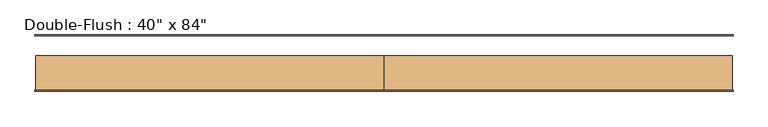
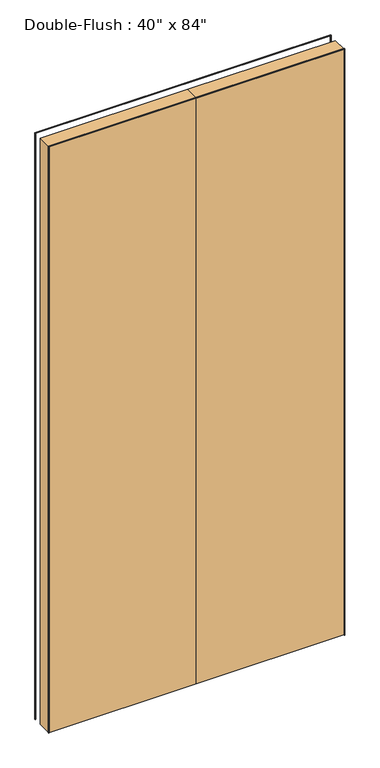
"""IFC4 building model written with IfcOpenShell, lengths in millimetres: door geometry."""

import ifcopenshell
import ifcopenshell.guid

model = None  # the IFC model being written
_history = None  # IfcOwnerHistory: only IFC2X3 demands one
_inside = {}  # id of a spatial element -> (the spatial element, [elements in it])
_under = {}  # id of a project, library or spatial element -> (it, [spatial elements below it])
_declared = {}  # id of a project -> (the project, [libraries it declares])
_typed = {}  # id of a type object -> (the type object, [elements of that type])
_made_of = {}  # id of a material, layer set ... -> (it, [elements and type objects made of it])


def new_model(schema):
    """Start an empty IFC model of exactly this schema.

    Asked for "IFC4X3", IfcOpenShell would pick the latest addendum, in which some entities
    have other attributes; the version numbers below select the first issue.
    IFC2X3 requires an IfcOwnerHistory on every rooted entity: one is made here for all.
    """
    global model, _history
    if schema == "IFC4X3":
        model = ifcopenshell.file(schema_version=(4, 3, 0, 0))
    else:
        model = ifcopenshell.file(schema=schema)
    _inside.clear()
    _under.clear()
    _declared.clear()
    _typed.clear()
    _made_of.clear()
    _history = None
    if model.schema == "IFC2X3":
        org = make("IfcOrganization", Name="unknown")
        user = make(
            "IfcPersonAndOrganization",
            ThePerson=make("IfcPerson", FamilyName="unknown"),
            TheOrganization=org,
        )
        app = make(
            "IfcApplication",
            ApplicationDeveloper=org,
            Version="unknown",
            ApplicationFullName="unknown",
            ApplicationIdentifier="unknown",
        )
        _history = make(
            "IfcOwnerHistory",
            OwningUser=user,
            OwningApplication=app,
            ChangeAction="ADDED",
            CreationDate=0,
        )
    return model


def make(cls, **values):
    """One entity of the class cls with the attributes given. An attribute that is None is left unset."""
    return model.create_entity(
        cls, **{name: value for name, value in values.items() if value is not None}
    )


def rooted(cls, **values):
    """An entity with a GlobalId (a new one), such as an element, a storey or a relation."""
    return make(cls, GlobalId=ifcopenshell.guid.new(), OwnerHistory=_history, **values)


def si_unit(unit_type, name, prefix=None):
    """IfcSIUnit, for example si_unit("LENGTHUNIT", "METRE", prefix="MILLI")."""
    return make("IfcSIUnit", UnitType=unit_type, Prefix=prefix, Name=name)


def assignment(units):
    """IfcUnitAssignment: the units of a project."""
    return None if units is None else make("IfcUnitAssignment", Units=units)


def point(xyz):
    """IfcCartesianPoint."""
    return None if xyz is None else make("IfcCartesianPoint", Coordinates=xyz)


def direction(xyz):
    """IfcDirection."""
    return None if xyz is None else make("IfcDirection", DirectionRatios=xyz)


def frame(location, z_axis=None, x_axis=None):
    """IfcAxis2Placement3D, a coordinate frame: its origin and axes. An axis left out is left unset."""
    return make(
        "IfcAxis2Placement3D",
        Location=point(location),
        Axis=direction(z_axis),
        RefDirection=direction(x_axis),
    )


def origin():
    """The frame at (0, 0, 0) with its axes left unset."""
    return frame((0.0, 0.0, 0.0))


def origin_with_axes():
    """The frame at (0, 0, 0) with the z axis (0, 0, 1) and the x axis (1, 0, 0) written out."""
    return frame((0.0, 0.0, 0.0), z_axis=(0.0, 0.0, 1.0), x_axis=(1.0, 0.0, 0.0))


def place(relative_to, where):
    """IfcLocalPlacement: puts the frame where relative to a parent placement (None: the world)."""
    return make(
        "IfcLocalPlacement", PlacementRelTo=relative_to, RelativePlacement=where
    )


def context(
    kind, dimensions, precision=None, world=None, true_north=None, identifier=None
):
    """IfcGeometricRepresentationContext, for example the 3D "Model" context."""
    return make(
        "IfcGeometricRepresentationContext",
        ContextIdentifier=identifier,
        ContextType=kind,
        CoordinateSpaceDimension=dimensions,
        Precision=precision,
        WorldCoordinateSystem=world,
        TrueNorth=true_north,
    )


def project(units=None, contexts=None):
    """IfcProject with its units and contexts."""
    return rooted(
        "IfcProject",
        Name="project",
        RepresentationContexts=contexts,
        UnitsInContext=assignment(units),
    )


def spatial(cls, under=None, at=None, **own):
    """A site, building, storey or space (cls), placed at a placement, below another one or the project."""
    s = rooted(cls, ObjectPlacement=at, **own)
    if under is not None:
        _under.setdefault(under.id(), (under, []))[1].append(s)
    return s


def polyline(points):
    """IfcPolyline through the points."""
    return make("IfcPolyline", Points=[point(p) for p in points])


def outline(outer, holes=None, kind="AREA"):
    """IfcArbitraryClosedProfileDef: a profile drawn as a closed curve; with holes, ...WithVoids."""
    if holes is None:
        return make("IfcArbitraryClosedProfileDef", ProfileType=kind, OuterCurve=outer)
    return make(
        "IfcArbitraryProfileDefWithVoids",
        ProfileType=kind,
        OuterCurve=outer,
        InnerCurves=holes,
    )


def extrude(swept, where, along, depth):
    """IfcExtrudedAreaSolid: the profile swept, set in the frame where, extruded along a direction by depth."""
    return make(
        "IfcExtrudedAreaSolid",
        SweptArea=swept,
        Position=where,
        ExtrudedDirection=direction(along),
        Depth=depth,
    )


def shape(context_of_items, identifier, shape_type, items):
    """IfcShapeRepresentation: the items that make up one representation, for example the "Body"."""
    return make(
        "IfcShapeRepresentation",
        ContextOfItems=context_of_items,
        RepresentationIdentifier=identifier,
        RepresentationType=shape_type,
        Items=items,
    )


def source(mapping_origin, context_of_items, identifier, shape_type, items):
    """IfcRepresentationMap: a shape defined once, which mapped items show again and again."""
    return make(
        "IfcRepresentationMap",
        MappingOrigin=mapping_origin,
        MappedRepresentation=shape(context_of_items, identifier, shape_type, items),
    )


def transform(
    local_origin,
    x_axis=None,
    y_axis=None,
    z_axis=None,
    scale=None,
    scale2=None,
    scale3=None,
    uniform=True,
):
    """IfcCartesianTransformationOperator3D, or its non-uniform kind. x_axis, y_axis, z_axis: its Axis1, 2, 3."""
    if uniform:
        return make(
            "IfcCartesianTransformationOperator3D",
            Axis1=direction(x_axis),
            Axis2=direction(y_axis),
            LocalOrigin=point(local_origin),
            Scale=scale,
            Axis3=direction(z_axis),
        )
    return make(
        "IfcCartesianTransformationOperator3DnonUniform",
        Axis1=direction(x_axis),
        Axis2=direction(y_axis),
        LocalOrigin=point(local_origin),
        Scale=scale,
        Axis3=direction(z_axis),
        Scale2=scale2,
        Scale3=scale3,
    )


def mapped(mapping_source, mapping_target):
    """IfcMappedItem: shows the shape of a source again, moved by a transform."""
    return make(
        "IfcMappedItem", MappingSource=mapping_source, MappingTarget=mapping_target
    )


def made_of(thing, what):
    """Note that an element or type object is made of a material, layer set ...; save() writes the relation."""
    if what is not None:
        _made_of.setdefault(what.id(), (what, []))[1].append(thing)
    return thing


def element(
    cls,
    number,
    at=None,
    inside=None,
    cuts=None,
    type_object=None,
    material=None,
    context=None,
    identifier="Body",
    shape_type=None,
    held_by="IfcProductDefinitionShape",
    body=None,
    shapes=None,
    **own,
):
    """One element of the class cls, such as IfcWall. Its Tag is "e" and its number.

    at: its placement. inside: the storey or other place that contains it. cuts: it is an
    opening in that element (IfcRelVoidsElement). A single representation is given by context,
    identifier, shape_type and body (its items); several are given by shapes. held_by: the class
    of the entity that holds the representations. save() writes the other relations.
    """
    e = rooted(cls, Tag="e%d" % number, ObjectPlacement=at, **own)
    if body is not None:
        shapes = [shape(context, identifier, shape_type, body)]
    if shapes is not None:
        e.Representation = make(held_by, Representations=shapes)
    if inside is not None:
        _inside.setdefault(inside.id(), (inside, []))[1].append(e)
    if cuts is not None:
        rooted(
            "IfcRelVoidsElement", RelatingBuildingElement=cuts, RelatedOpeningElement=e
        )
    if type_object is not None:
        _typed.setdefault(type_object.id(), (type_object, []))[1].append(e)
    return made_of(e, material)


def aggregate(whole, parts):
    """IfcRelAggregates: a whole, such as a stair, and the parts it consists of."""
    return rooted("IfcRelAggregates", RelatingObject=whole, RelatedObjects=parts)


def save(model, path):
    """Write the relations noted so far, then the file.

    IfcRelAggregates (storeys below a building ...), IfcRelContainedInSpatialStructure (elements
    in a storey), IfcRelDefinesByType, IfcRelAssociatesMaterial and IfcRelDeclares: one each for
    every whole, place, type object, material and project.
    """
    for whole, parts in _under.values():
        aggregate(whole, parts)
    for where, things in _inside.values():
        rooted(
            "IfcRelContainedInSpatialStructure",
            RelatedElements=things,
            RelatingStructure=where,
        )
    for kind, things in _typed.values():
        rooted("IfcRelDefinesByType", RelatedObjects=things, RelatingType=kind)
    for what, things in _made_of.values():
        rooted("IfcRelAssociatesMaterial", RelatedObjects=things, RelatingMaterial=what)
    for by, libraries in _declared.values():
        rooted("IfcRelDeclares", RelatingContext=by, RelatedDefinitions=libraries)
    model.write(path)


def door_b060f29f(model_context):
    return source(origin(), model_context, "Body", "SweptSolid", [
        extrude(outline(polyline([(0.0, -39.6875), (0.0, 11.1125), (508.0, 11.1125), (508.0, -39.6875), (0.0, -39.6875)])), origin_with_axes(), (0.0, 0.0, 1.0), 2133.6),
        extrude(outline(polyline([(-508.0, -39.6875), (-508.0, 11.1125), (0.0, 11.1125), (0.0, -39.6875), (-508.0, -39.6875)])), origin_with_axes(), (0.0, 0.0, 1.0), 2133.6),
        extrude(outline(polyline([(2133.6, -508.0), (2133.6, 508.0), (0.0, 508.0), (0.0, 509.5875), (2135.1875, 509.5875), (2135.1875, -509.5875), (0.0, -509.5875), (0.0, -508.0), (2133.6, -508.0)])), frame((0.0, 39.6875, 0.0), z_axis=(0.0, 1.0, 0.0), x_axis=(0.0, 0.0, 1.0)), (0.0, 0.0, 1.0), 1.5875),
        extrude(outline(polyline([(2133.6, -508.0), (2133.6, 508.0), (0.0, 508.0), (0.0, 509.5875), (2135.1875, 509.5875), (2135.1875, -509.5875), (0.0, -509.5875), (0.0, -508.0), (2133.6, -508.0)])), frame((0.0, -41.275, 0.0), z_axis=(0.0, 1.0, 0.0), x_axis=(0.0, 0.0, 1.0)), (0.0, 0.0, 1.0), 1.5875),
    ])


if __name__ == "__main__":
    model = new_model("IFC4")
    model_context = context("Model", 3, world=origin())
    ifc_project = project(units=[si_unit("LENGTHUNIT", "METRE", prefix="MILLI")], contexts=[model_context])
    site = spatial("IfcSite", under=ifc_project)
    building = spatial("IfcBuilding", under=site)
    placement = place(None, origin())
    door_shape = door_b060f29f(model_context)
    element("IfcDoor", 1, ObjectType="Double-Flush : 40\" x 84\"", at=placement, inside=building, context=model_context, shape_type="MappedRepresentation", body=[
        mapped(door_shape, transform((0.0, 0.0, 0.0), x_axis=(1.0, 0.0, 0.0), y_axis=(0.0, 1.0, 0.0), z_axis=(0.0, 0.0, 1.0))),
    ])
    save(model, "model.ifc")

# Revit data of these elements
# Type "Double-Flush : 40\" x 84\""
#   Type Mark = "41"
#   Assembly Code = "C1020"
#   Thickness = 0' - 2"
#   Height = 7' - 0"
#   Trim Projection Ext = 0' - 0 1/16"
#   Trim Projection Int = 0' - 0 1/16"
#   Trim Width = 0' - 0 1/16"
#   Width = 3' - 4"
#   Door Material = Door - Panel
#   Frame Material = Door - Frame
#   Function = (empty or 0)
#   Wall Closure = (empty or 0)
# Element 1 (IfcDoor, "Double-Flush : 40\" x 84\"")
#   Materials on its faces: "Door - Frame", "Door - Panel"
# Materials
#   "Door - Panel": class "Wood", colour RGB 210 159 95, transparency 0
#   "Door - Frame": class "Miscellaneous", colour RGB 118 70 51, transparency 0
